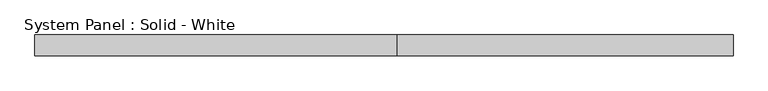
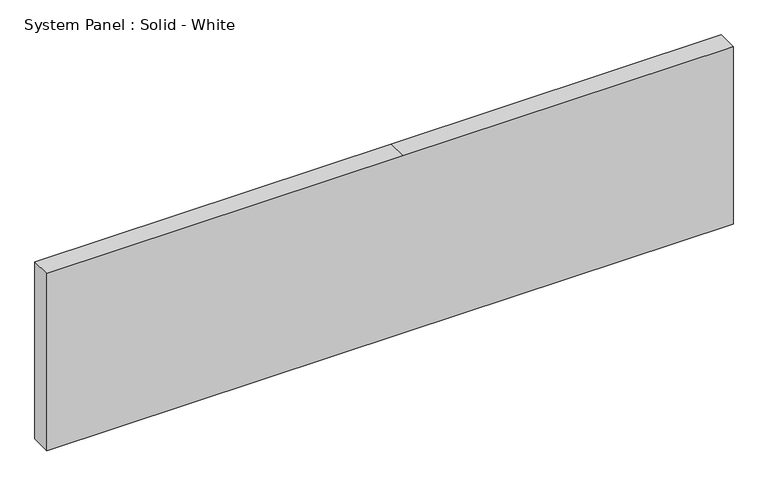
"""IFC4 building model written with IfcOpenShell, lengths in millimetres: plate geometry, System Panel : Solid - White."""

import ifcopenshell
import ifcopenshell.guid

model = None  # the IFC model being written
_history = None  # IfcOwnerHistory: only IFC2X3 demands one
_inside = {}  # id of a spatial element -> (the spatial element, [elements in it])
_under = {}  # id of a project, library or spatial element -> (it, [spatial elements below it])
_declared = {}  # id of a project -> (the project, [libraries it declares])
_typed = {}  # id of a type object -> (the type object, [elements of that type])
_made_of = {}  # id of a material, layer set ... -> (it, [elements and type objects made of it])


def new_model(schema):
    """Start an empty IFC model of exactly this schema.

    Asked for "IFC4X3", IfcOpenShell would pick the latest addendum, in which some entities
    have other attributes; the version numbers below select the first issue.
    IFC2X3 requires an IfcOwnerHistory on every rooted entity: one is made here for all.
    """
    global model, _history
    if schema == "IFC4X3":
        model = ifcopenshell.file(schema_version=(4, 3, 0, 0))
    else:
        model = ifcopenshell.file(schema=schema)
    _inside.clear()
    _under.clear()
    _declared.clear()
    _typed.clear()
    _made_of.clear()
    _history = None
    if model.schema == "IFC2X3":
        org = make("IfcOrganization", Name="unknown")
        user = make(
            "IfcPersonAndOrganization",
            ThePerson=make("IfcPerson", FamilyName="unknown"),
            TheOrganization=org,
        )
        app = make(
            "IfcApplication",
            ApplicationDeveloper=org,
            Version="unknown",
            ApplicationFullName="unknown",
            ApplicationIdentifier="unknown",
        )
        _history = make(
            "IfcOwnerHistory",
            OwningUser=user,
            OwningApplication=app,
            ChangeAction="ADDED",
            CreationDate=0,
        )
    return model


def make(cls, **values):
    """One entity of the class cls with the attributes given. An attribute that is None is left unset."""
    return model.create_entity(
        cls, **{name: value for name, value in values.items() if value is not None}
    )


def rooted(cls, **values):
    """An entity with a GlobalId (a new one), such as an element, a storey or a relation."""
    return make(cls, GlobalId=ifcopenshell.guid.new(), OwnerHistory=_history, **values)


def si_unit(unit_type, name, prefix=None):
    """IfcSIUnit, for example si_unit("LENGTHUNIT", "METRE", prefix="MILLI")."""
    return make("IfcSIUnit", UnitType=unit_type, Prefix=prefix, Name=name)


def assignment(units):
    """IfcUnitAssignment: the units of a project."""
    return None if units is None else make("IfcUnitAssignment", Units=units)


def point(xyz):
    """IfcCartesianPoint."""
    return None if xyz is None else make("IfcCartesianPoint", Coordinates=xyz)


def direction(xyz):
    """IfcDirection."""
    return None if xyz is None else make("IfcDirection", DirectionRatios=xyz)


def frame(location, z_axis=None, x_axis=None):
    """IfcAxis2Placement3D, a coordinate frame: its origin and axes. An axis left out is left unset."""
    return make(
        "IfcAxis2Placement3D",
        Location=point(location),
        Axis=direction(z_axis),
        RefDirection=direction(x_axis),
    )


def origin():
    """The frame at (0, 0, 0) with its axes left unset."""
    return frame((0.0, 0.0, 0.0))


def place(relative_to, where):
    """IfcLocalPlacement: puts the frame where relative to a parent placement (None: the world)."""
    return make(
        "IfcLocalPlacement", PlacementRelTo=relative_to, RelativePlacement=where
    )


def context(
    kind, dimensions, precision=None, world=None, true_north=None, identifier=None
):
    """IfcGeometricRepresentationContext, for example the 3D "Model" context."""
    return make(
        "IfcGeometricRepresentationContext",
        ContextIdentifier=identifier,
        ContextType=kind,
        CoordinateSpaceDimension=dimensions,
        Precision=precision,
        WorldCoordinateSystem=world,
        TrueNorth=true_north,
    )


def project(units=None, contexts=None):
    """IfcProject with its units and contexts."""
    return rooted(
        "IfcProject",
        Name="project",
        RepresentationContexts=contexts,
        UnitsInContext=assignment(units),
    )


def spatial(cls, under=None, at=None, **own):
    """A site, building, storey or space (cls), placed at a placement, below another one or the project."""
    s = rooted(cls, ObjectPlacement=at, **own)
    if under is not None:
        _under.setdefault(under.id(), (under, []))[1].append(s)
    return s


def polyline(points):
    """IfcPolyline through the points."""
    return make("IfcPolyline", Points=[point(p) for p in points])


def outline(outer, holes=None, kind="AREA"):
    """IfcArbitraryClosedProfileDef: a profile drawn as a closed curve; with holes, ...WithVoids."""
    if holes is None:
        return make("IfcArbitraryClosedProfileDef", ProfileType=kind, OuterCurve=outer)
    return make(
        "IfcArbitraryProfileDefWithVoids",
        ProfileType=kind,
        OuterCurve=outer,
        InnerCurves=holes,
    )


def extrude(swept, where, along, depth):
    """IfcExtrudedAreaSolid: the profile swept, set in the frame where, extruded along a direction by depth."""
    return make(
        "IfcExtrudedAreaSolid",
        SweptArea=swept,
        Position=where,
        ExtrudedDirection=direction(along),
        Depth=depth,
    )


def shape(context_of_items, identifier, shape_type, items):
    """IfcShapeRepresentation: the items that make up one representation, for example the "Body"."""
    return make(
        "IfcShapeRepresentation",
        ContextOfItems=context_of_items,
        RepresentationIdentifier=identifier,
        RepresentationType=shape_type,
        Items=items,
    )


def source(mapping_origin, context_of_items, identifier, shape_type, items):
    """IfcRepresentationMap: a shape defined once, which mapped items show again and again."""
    return make(
        "IfcRepresentationMap",
        MappingOrigin=mapping_origin,
        MappedRepresentation=shape(context_of_items, identifier, shape_type, items),
    )


def transform(
    local_origin,
    x_axis=None,
    y_axis=None,
    z_axis=None,
    scale=None,
    scale2=None,
    scale3=None,
    uniform=True,
):
    """IfcCartesianTransformationOperator3D, or its non-uniform kind. x_axis, y_axis, z_axis: its Axis1, 2, 3."""
    if uniform:
        return make(
            "IfcCartesianTransformationOperator3D",
            Axis1=direction(x_axis),
            Axis2=direction(y_axis),
            LocalOrigin=point(local_origin),
            Scale=scale,
            Axis3=direction(z_axis),
        )
    return make(
        "IfcCartesianTransformationOperator3DnonUniform",
        Axis1=direction(x_axis),
        Axis2=direction(y_axis),
        LocalOrigin=point(local_origin),
        Scale=scale,
        Axis3=direction(z_axis),
        Scale2=scale2,
        Scale3=scale3,
    )


def mapped(mapping_source, mapping_target):
    """IfcMappedItem: shows the shape of a source again, moved by a transform."""
    return make(
        "IfcMappedItem", MappingSource=mapping_source, MappingTarget=mapping_target
    )


def made_of(thing, what):
    """Note that an element or type object is made of a material, layer set ...; save() writes the relation."""
    if what is not None:
        _made_of.setdefault(what.id(), (what, []))[1].append(thing)
    return thing


def element(
    cls,
    number,
    at=None,
    inside=None,
    cuts=None,
    type_object=None,
    material=None,
    context=None,
    identifier="Body",
    shape_type=None,
    held_by="IfcProductDefinitionShape",
    body=None,
    shapes=None,
    **own,
):
    """One element of the class cls, such as IfcWall. Its Tag is "e" and its number.

    at: its placement. inside: the storey or other place that contains it. cuts: it is an
    opening in that element (IfcRelVoidsElement). A single representation is given by context,
    identifier, shape_type and body (its items); several are given by shapes. held_by: the class
    of the entity that holds the representations. save() writes the other relations.
    """
    e = rooted(cls, Tag="e%d" % number, ObjectPlacement=at, **own)
    if body is not None:
        shapes = [shape(context, identifier, shape_type, body)]
    if shapes is not None:
        e.Representation = make(held_by, Representations=shapes)
    if inside is not None:
        _inside.setdefault(inside.id(), (inside, []))[1].append(e)
    if cuts is not None:
        rooted(
            "IfcRelVoidsElement", RelatingBuildingElement=cuts, RelatedOpeningElement=e
        )
    if type_object is not None:
        _typed.setdefault(type_object.id(), (type_object, []))[1].append(e)
    return made_of(e, material)


def aggregate(whole, parts):
    """IfcRelAggregates: a whole, such as a stair, and the parts it consists of."""
    return rooted("IfcRelAggregates", RelatingObject=whole, RelatedObjects=parts)


def save(model, path):
    """Write the relations noted so far, then the file.

    IfcRelAggregates (storeys below a building ...), IfcRelContainedInSpatialStructure (elements
    in a storey), IfcRelDefinesByType, IfcRelAssociatesMaterial and IfcRelDeclares: one each for
    every whole, place, type object, material and project.
    """
    for whole, parts in _under.values():
        aggregate(whole, parts)
    for where, things in _inside.values():
        rooted(
            "IfcRelContainedInSpatialStructure",
            RelatedElements=things,
            RelatingStructure=where,
        )
    for kind, things in _typed.values():
        rooted("IfcRelDefinesByType", RelatedObjects=things, RelatingType=kind)
    for what, things in _made_of.values():
        rooted("IfcRelAssociatesMaterial", RelatedObjects=things, RelatingMaterial=what)
    for by, libraries in _declared.values():
        rooted("IfcRelDeclares", RelatingContext=by, RelatedDefinitions=libraries)
    model.write(path)


def system_panel_solid_white_6903a38c(model_context):
    return source(origin(), model_context, "Body", "SweptSolid", [
        extrude(outline(polyline([(0.0, -1057.7285714), (0.0, 40.8214286), (0.0, 1057.7285714), (577.85, 1057.7285714), (577.85, 40.8214286), (577.85, -1057.7285714), (0.0, -1057.7285714)])), frame((0.0, -19.05, 0.0), z_axis=(0.0, 1.0, 0.0), x_axis=(0.0, 0.0, 1.0)), (0.0, 0.0, 1.0), 63.5),
    ])


if __name__ == "__main__":
    model = new_model("IFC4")
    model_context = context("Model", 3, world=origin())
    ifc_project = project(units=[si_unit("LENGTHUNIT", "METRE", prefix="MILLI")], contexts=[model_context])
    site = spatial("IfcSite", under=ifc_project)
    building = spatial("IfcBuilding", under=site)
    placement = place(None, origin())
    system_panel_solid_white_shape = system_panel_solid_white_6903a38c(model_context)
    element("IfcPlate", 1, ObjectType="System Panel : Solid - White", at=placement, inside=building, context=model_context, shape_type="MappedRepresentation", body=[
        mapped(system_panel_solid_white_shape, transform((0.0, 0.0, 0.0), x_axis=(1.0, 0.0, 0.0), y_axis=(0.0, 1.0, 0.0), z_axis=(0.0, 0.0, 1.0))),
    ])
    save(model, "model.ifc")

# Revit data of these elements
# Element 1 (IfcPlate, "System Panel : Solid - White")
#   Materials on its faces: "White Panel"
# Materials
#   "White Panel": class "Unassigned", colour RGB 255 255 255, transparency 0
